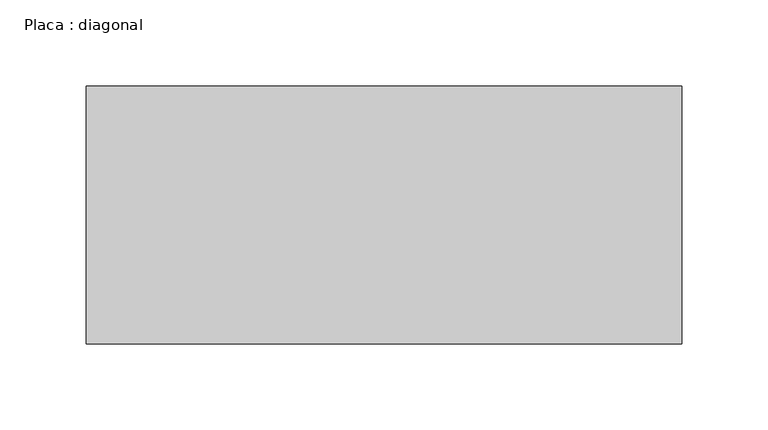
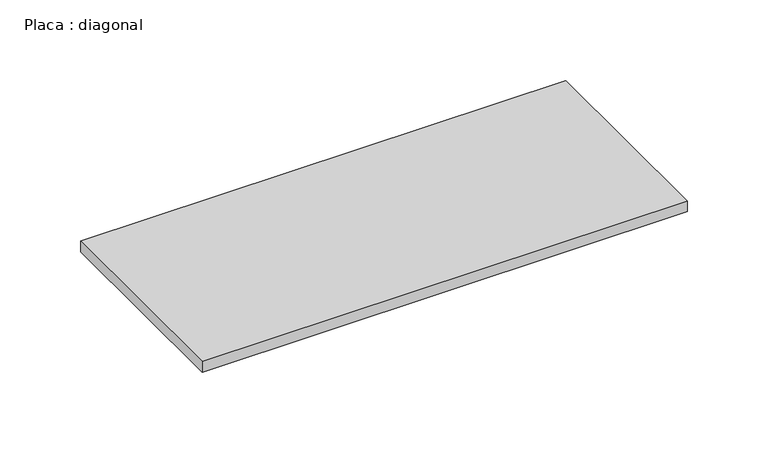
"""IFC4 building model written with IfcOpenShell, lengths in millimetres: beam geometry, Placa : diagonal."""

from ifc_helpers import new_model, si_unit, frame, origin, place, context, project, spatial, polyline, outline, extrude, source, transform, mapped, element, save


def placa_diagonal_a71479e9(model_context):
    return source(origin(), model_context, "Body", "SweptSolid", [
        extrude(outline(polyline([(161.178496, 75.0), (161.178496, -75.0), (-185.3041805, -75.0), (-185.3041805, 75.0), (161.178496, 75.0)])), frame((0.0, 0.0, -4.0), z_axis=(0.0, 0.0, 1.0), x_axis=(1.0, 0.0, 0.0)), (0.0, 0.0, 1.0), 8.0),
    ])


if __name__ == "__main__":
    model = new_model("IFC4")
    model_context = context("Model", 3, world=origin())
    ifc_project = project(units=[si_unit("LENGTHUNIT", "METRE", prefix="MILLI")], contexts=[model_context])
    site = spatial("IfcSite", under=ifc_project)
    building = spatial("IfcBuilding", under=site)
    placement = place(None, origin())
    placa_diagonal_shape = placa_diagonal_a71479e9(model_context)
    element("IfcBeam", 1, ObjectType="Placa : diagonal", at=placement, inside=building, context=model_context, shape_type="MappedRepresentation", body=[
        mapped(placa_diagonal_shape, transform((0.0, 0.0, 0.0), x_axis=(1.0, 0.0, 0.0), y_axis=(0.0, 1.0, 0.0), z_axis=(0.0, 0.0, 1.0))),
    ])
    save(model, "model.ifc")

# Revit data of these elements
# Type "Placa : diagonal"
#   W = 0
#   Length [instance default] = 1.50 m
#   b = 0.15 m
#   d = 0.008 m
#   A = 0 m²
#   Structural Material [instance default] = Aço, 45-345
# Element 1 (IfcBeam, "Placa : diagonal")
#   Materials on its faces: "Aço, 45-345"
# Materials
#   "Aço, 45-345": class "Metal", colour RGB 247 247 247, transparency 0, Description = "Aço 345 MPa", Cost = 0
